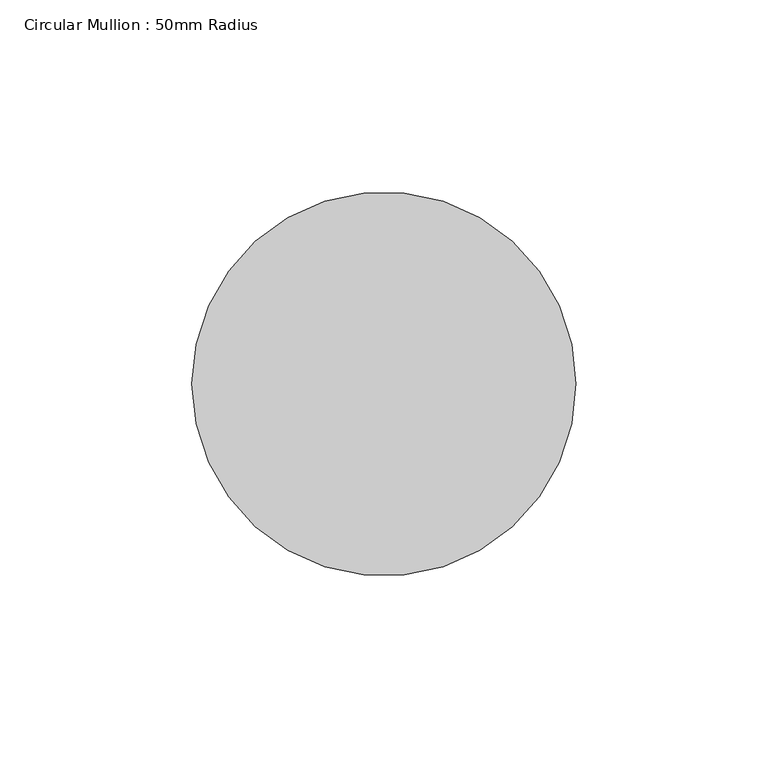
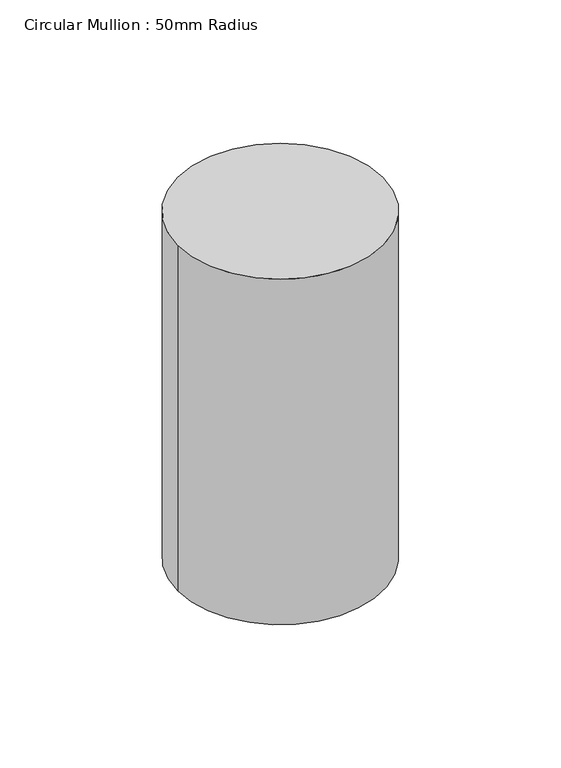
"""IFC4 building model written with IfcOpenShell, lengths in millimetres: member geometry, Circular Mullion : 50mm Radius."""

from ifc_helpers import new_model, si_unit, point, frame, origin, origin_2d, place, context, project, spatial, circle_curve, trimmed, segment, composite_curve, outline, extrude, source, transform, mapped, element, save


def circular_mullion_50mm_radius_d24bb71c(model_context):
    return source(origin(), model_context, "Body", "SweptSolid", [
        extrude(outline(composite_curve([segment(trimmed(circle_curve(origin_2d(), 50.0), [point((50.0, 0.0))], [point((-50.0, 0.0))], False, "CARTESIAN"), True, "CONTINUOUS"), segment(trimmed(circle_curve(origin_2d(), 50.0), [point((-50.0, 0.0))], [point((50.0, 0.0))], False, "CARTESIAN"), True, "CONTINUOUS")], self_intersect=False)), frame((0.0, 0.0, -177.9848542), z_axis=(0.0, 0.0, 1.0), x_axis=(1.0, 0.0, 0.0)), (0.0, 0.0, 1.0), 177.9848542),
    ])


if __name__ == "__main__":
    model = new_model("IFC4")
    model_context = context("Model", 3, world=origin())
    ifc_project = project(units=[si_unit("LENGTHUNIT", "METRE", prefix="MILLI")], contexts=[model_context])
    site = spatial("IfcSite", under=ifc_project)
    building = spatial("IfcBuilding", under=site)
    placement = place(None, origin())
    circular_mullion_50mm_radius_shape = circular_mullion_50mm_radius_d24bb71c(model_context)
    element("IfcMember", 1, ObjectType="Circular Mullion : 50mm Radius", at=placement, inside=building, context=model_context, shape_type="MappedRepresentation", body=[
        mapped(circular_mullion_50mm_radius_shape, transform((0.0, 0.0, 0.0), x_axis=(1.0, 0.0, 0.0), y_axis=(0.0, 1.0, 0.0), z_axis=(0.0, 0.0, 1.0))),
    ])
    save(model, "model.ifc")

# Revit data of these elements
# Type "Circular Mullion : 50mm Radius"
#   built-in parameter 1007350 = 0.164042 (stored number, unit not read)
# Element 1 (IfcMember, "Circular Mullion : 50mm Radius")
#   Materials on its faces: "Aluminium"
# Materials
#   "Aluminium": class "Metal", colour RGB 247 247 247, transparency 0, Description = "Aluminium 6061", Cost = 0
